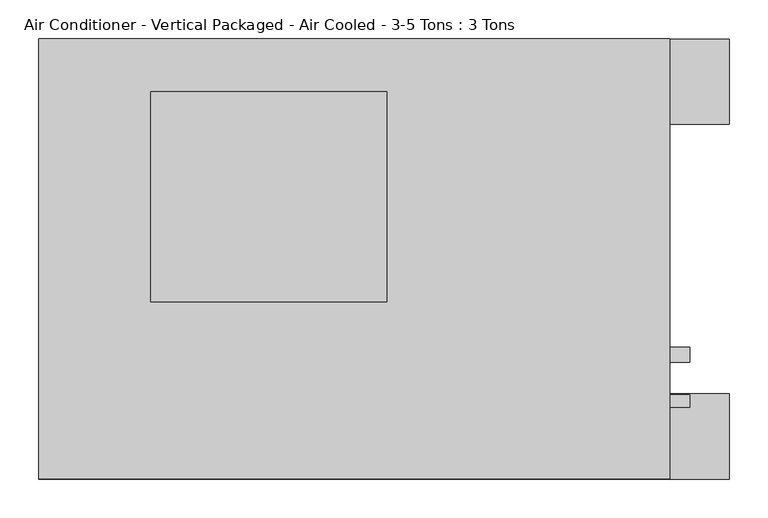
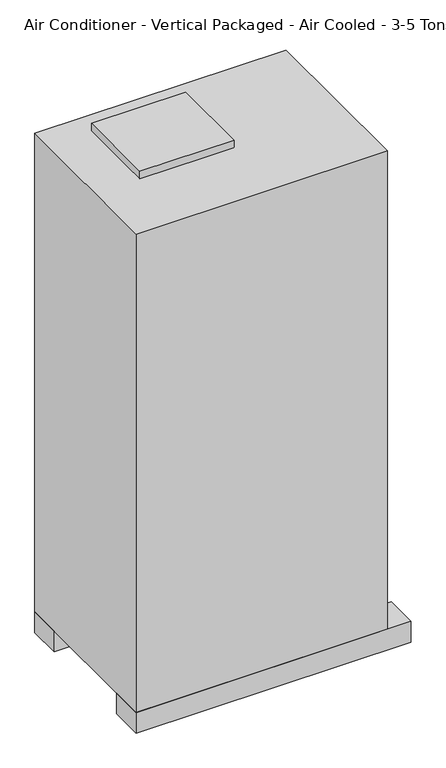
"""IFC4 building model written with IfcOpenShell, lengths in millimetres: proxy geometry, Air Conditioner - Vertical Packaged - Air Cooled - 3-5 Tons : 3 Tons."""

import ifcopenshell
import ifcopenshell.guid

model = None  # the IFC model being written
_history = None  # IfcOwnerHistory: only IFC2X3 demands one
_inside = {}  # id of a spatial element -> (the spatial element, [elements in it])
_under = {}  # id of a project, library or spatial element -> (it, [spatial elements below it])
_declared = {}  # id of a project -> (the project, [libraries it declares])
_typed = {}  # id of a type object -> (the type object, [elements of that type])
_made_of = {}  # id of a material, layer set ... -> (it, [elements and type objects made of it])


def new_model(schema):
    """Start an empty IFC model of exactly this schema.

    Asked for "IFC4X3", IfcOpenShell would pick the latest addendum, in which some entities
    have other attributes; the version numbers below select the first issue.
    IFC2X3 requires an IfcOwnerHistory on every rooted entity: one is made here for all.
    """
    global model, _history
    if schema == "IFC4X3":
        model = ifcopenshell.file(schema_version=(4, 3, 0, 0))
    else:
        model = ifcopenshell.file(schema=schema)
    _inside.clear()
    _under.clear()
    _declared.clear()
    _typed.clear()
    _made_of.clear()
    _history = None
    if model.schema == "IFC2X3":
        org = make("IfcOrganization", Name="unknown")
        user = make(
            "IfcPersonAndOrganization",
            ThePerson=make("IfcPerson", FamilyName="unknown"),
            TheOrganization=org,
        )
        app = make(
            "IfcApplication",
            ApplicationDeveloper=org,
            Version="unknown",
            ApplicationFullName="unknown",
            ApplicationIdentifier="unknown",
        )
        _history = make(
            "IfcOwnerHistory",
            OwningUser=user,
            OwningApplication=app,
            ChangeAction="ADDED",
            CreationDate=0,
        )
    return model


def make(cls, **values):
    """One entity of the class cls with the attributes given. An attribute that is None is left unset."""
    return model.create_entity(
        cls, **{name: value for name, value in values.items() if value is not None}
    )


def rooted(cls, **values):
    """An entity with a GlobalId (a new one), such as an element, a storey or a relation."""
    return make(cls, GlobalId=ifcopenshell.guid.new(), OwnerHistory=_history, **values)


def si_unit(unit_type, name, prefix=None):
    """IfcSIUnit, for example si_unit("LENGTHUNIT", "METRE", prefix="MILLI")."""
    return make("IfcSIUnit", UnitType=unit_type, Prefix=prefix, Name=name)


def assignment(units):
    """IfcUnitAssignment: the units of a project."""
    return None if units is None else make("IfcUnitAssignment", Units=units)


def point(xyz):
    """IfcCartesianPoint."""
    return None if xyz is None else make("IfcCartesianPoint", Coordinates=xyz)


def direction(xyz):
    """IfcDirection."""
    return None if xyz is None else make("IfcDirection", DirectionRatios=xyz)


def frame(location, z_axis=None, x_axis=None):
    """IfcAxis2Placement3D, a coordinate frame: its origin and axes. An axis left out is left unset."""
    return make(
        "IfcAxis2Placement3D",
        Location=point(location),
        Axis=direction(z_axis),
        RefDirection=direction(x_axis),
    )


def frame_2d(location, x_axis=None):
    """IfcAxis2Placement2D, a coordinate frame in the plane: its origin and x axis."""
    return make(
        "IfcAxis2Placement2D", Location=point(location), RefDirection=direction(x_axis)
    )


def origin():
    """The frame at (0, 0, 0) with its axes left unset."""
    return frame((0.0, 0.0, 0.0))


def origin_with_axes():
    """The frame at (0, 0, 0) with the z axis (0, 0, 1) and the x axis (1, 0, 0) written out."""
    return frame((0.0, 0.0, 0.0), z_axis=(0.0, 0.0, 1.0), x_axis=(1.0, 0.0, 0.0))


def place(relative_to, where):
    """IfcLocalPlacement: puts the frame where relative to a parent placement (None: the world)."""
    return make(
        "IfcLocalPlacement", PlacementRelTo=relative_to, RelativePlacement=where
    )


def context(
    kind, dimensions, precision=None, world=None, true_north=None, identifier=None
):
    """IfcGeometricRepresentationContext, for example the 3D "Model" context."""
    return make(
        "IfcGeometricRepresentationContext",
        ContextIdentifier=identifier,
        ContextType=kind,
        CoordinateSpaceDimension=dimensions,
        Precision=precision,
        WorldCoordinateSystem=world,
        TrueNorth=true_north,
    )


def project(units=None, contexts=None):
    """IfcProject with its units and contexts."""
    return rooted(
        "IfcProject",
        Name="project",
        RepresentationContexts=contexts,
        UnitsInContext=assignment(units),
    )


def spatial(cls, under=None, at=None, **own):
    """A site, building, storey or space (cls), placed at a placement, below another one or the project."""
    s = rooted(cls, ObjectPlacement=at, **own)
    if under is not None:
        _under.setdefault(under.id(), (under, []))[1].append(s)
    return s


def polyline(points):
    """IfcPolyline through the points."""
    return make("IfcPolyline", Points=[point(p) for p in points])


def circle_curve(where, radius):
    """IfcCircle in the frame where."""
    return make("IfcCircle", Position=where, Radius=radius)


def trimmed(basis, trim1, trim2, sense, master):
    """IfcTrimmedCurve: the piece of a basis curve between two trims."""
    return make(
        "IfcTrimmedCurve",
        BasisCurve=basis,
        Trim1=trim1,
        Trim2=trim2,
        SenseAgreement=sense,
        MasterRepresentation=master,
    )


def segment(curve, same_sense, transition):
    """IfcCompositeCurveSegment."""
    return make(
        "IfcCompositeCurveSegment",
        Transition=transition,
        SameSense=same_sense,
        ParentCurve=curve,
    )


def composite_curve(segments, self_intersect=None):
    """IfcCompositeCurve: segments joined end to end."""
    return make("IfcCompositeCurve", Segments=segments, SelfIntersect=self_intersect)


def outline(outer, holes=None, kind="AREA"):
    """IfcArbitraryClosedProfileDef: a profile drawn as a closed curve; with holes, ...WithVoids."""
    if holes is None:
        return make("IfcArbitraryClosedProfileDef", ProfileType=kind, OuterCurve=outer)
    return make(
        "IfcArbitraryProfileDefWithVoids",
        ProfileType=kind,
        OuterCurve=outer,
        InnerCurves=holes,
    )


def extrude(swept, where, along, depth):
    """IfcExtrudedAreaSolid: the profile swept, set in the frame where, extruded along a direction by depth."""
    return make(
        "IfcExtrudedAreaSolid",
        SweptArea=swept,
        Position=where,
        ExtrudedDirection=direction(along),
        Depth=depth,
    )


def shape(context_of_items, identifier, shape_type, items):
    """IfcShapeRepresentation: the items that make up one representation, for example the "Body"."""
    return make(
        "IfcShapeRepresentation",
        ContextOfItems=context_of_items,
        RepresentationIdentifier=identifier,
        RepresentationType=shape_type,
        Items=items,
    )


def source(mapping_origin, context_of_items, identifier, shape_type, items):
    """IfcRepresentationMap: a shape defined once, which mapped items show again and again."""
    return make(
        "IfcRepresentationMap",
        MappingOrigin=mapping_origin,
        MappedRepresentation=shape(context_of_items, identifier, shape_type, items),
    )


def transform(
    local_origin,
    x_axis=None,
    y_axis=None,
    z_axis=None,
    scale=None,
    scale2=None,
    scale3=None,
    uniform=True,
):
    """IfcCartesianTransformationOperator3D, or its non-uniform kind. x_axis, y_axis, z_axis: its Axis1, 2, 3."""
    if uniform:
        return make(
            "IfcCartesianTransformationOperator3D",
            Axis1=direction(x_axis),
            Axis2=direction(y_axis),
            LocalOrigin=point(local_origin),
            Scale=scale,
            Axis3=direction(z_axis),
        )
    return make(
        "IfcCartesianTransformationOperator3DnonUniform",
        Axis1=direction(x_axis),
        Axis2=direction(y_axis),
        LocalOrigin=point(local_origin),
        Scale=scale,
        Axis3=direction(z_axis),
        Scale2=scale2,
        Scale3=scale3,
    )


def mapped(mapping_source, mapping_target):
    """IfcMappedItem: shows the shape of a source again, moved by a transform."""
    return make(
        "IfcMappedItem", MappingSource=mapping_source, MappingTarget=mapping_target
    )


def made_of(thing, what):
    """Note that an element or type object is made of a material, layer set ...; save() writes the relation."""
    if what is not None:
        _made_of.setdefault(what.id(), (what, []))[1].append(thing)
    return thing


def element(
    cls,
    number,
    at=None,
    inside=None,
    cuts=None,
    type_object=None,
    material=None,
    context=None,
    identifier="Body",
    shape_type=None,
    held_by="IfcProductDefinitionShape",
    body=None,
    shapes=None,
    **own,
):
    """One element of the class cls, such as IfcWall. Its Tag is "e" and its number.

    at: its placement. inside: the storey or other place that contains it. cuts: it is an
    opening in that element (IfcRelVoidsElement). A single representation is given by context,
    identifier, shape_type and body (its items); several are given by shapes. held_by: the class
    of the entity that holds the representations. save() writes the other relations.
    """
    e = rooted(cls, Tag="e%d" % number, ObjectPlacement=at, **own)
    if body is not None:
        shapes = [shape(context, identifier, shape_type, body)]
    if shapes is not None:
        e.Representation = make(held_by, Representations=shapes)
    if inside is not None:
        _inside.setdefault(inside.id(), (inside, []))[1].append(e)
    if cuts is not None:
        rooted(
            "IfcRelVoidsElement", RelatingBuildingElement=cuts, RelatedOpeningElement=e
        )
    if type_object is not None:
        _typed.setdefault(type_object.id(), (type_object, []))[1].append(e)
    return made_of(e, material)


def aggregate(whole, parts):
    """IfcRelAggregates: a whole, such as a stair, and the parts it consists of."""
    return rooted("IfcRelAggregates", RelatingObject=whole, RelatedObjects=parts)


def save(model, path):
    """Write the relations noted so far, then the file.

    IfcRelAggregates (storeys below a building ...), IfcRelContainedInSpatialStructure (elements
    in a storey), IfcRelDefinesByType, IfcRelAssociatesMaterial and IfcRelDeclares: one each for
    every whole, place, type object, material and project.
    """
    for whole, parts in _under.values():
        aggregate(whole, parts)
    for where, things in _inside.values():
        rooted(
            "IfcRelContainedInSpatialStructure",
            RelatedElements=things,
            RelatingStructure=where,
        )
    for kind, things in _typed.values():
        rooted("IfcRelDefinesByType", RelatedObjects=things, RelatingType=kind)
    for what, things in _made_of.values():
        rooted("IfcRelAssociatesMaterial", RelatedObjects=things, RelatingMaterial=what)
    for by, libraries in _declared.values():
        rooted("IfcRelDeclares", RelatingContext=by, RelatedDefinitions=libraries)
    model.write(path)


def air_conditioner_vertical_packaged_air_cooled_3_5_tons_3_tons_b39a03d3(model_context):
    return source(origin(), model_context, "Body", "SweptSolid", [
        extrude(outline(composite_curve([segment(trimmed(circle_curve(frame_2d((159.54375, 513.0601562)), 9.525), [point((150.01875, 513.0601562))], [point((169.06875, 513.0601562))], False, "CARTESIAN"), True, "CONTINUOUS"), segment(trimmed(circle_curve(frame_2d((159.54375, 513.0601562)), 9.525), [point((169.06875, 513.0601562))], [point((150.01875, 513.0601562))], False, "CARTESIAN"), True, "CONTINUOUS")], self_intersect=False)), frame((810.021875, 0.0, 0.0), z_axis=(1.0, 0.0, 0.0), x_axis=(0.0, 1.0, 0.0)), (0.0, 0.0, 1.0), 25.4),
        extrude(outline(polyline([(446.484375, 497.0343437), (446.484375, 227.060125), (143.4703125, 227.060125), (143.4703125, 497.0343437), (446.484375, 497.0343437)])), frame((0.0, 0.0, 1700.069625), z_axis=(0.0, 0.0, 1.0), x_axis=(1.0, 0.0, 0.0)), (0.0, 0.0, 1.0), 25.4),
        extrude(outline(composite_curve([segment(trimmed(circle_curve(frame_2d((454.3226562, 330.9500937)), 12.7), [point((441.6226562, 330.9500937))], [point((467.0226562, 330.9500937))], False, "CARTESIAN"), True, "CONTINUOUS"), segment(trimmed(circle_curve(frame_2d((454.3226562, 330.9500937)), 12.7), [point((467.0226562, 330.9500937))], [point((441.6226562, 330.9500937))], False, "CARTESIAN"), True, "CONTINUOUS")], self_intersect=False)), frame((784.621875, 0.0, 0.0), z_axis=(1.0, 0.0, 0.0), x_axis=(0.0, 1.0, 0.0)), (0.0, 0.0, 1.0), 25.4),
        extrude(outline(composite_curve([segment(trimmed(circle_curve(frame_2d((100.1117188, 170.2157187)), 6.35), [point((93.7617188, 170.2157187))], [point((106.4617188, 170.2157187))], False, "CARTESIAN"), True, "CONTINUOUS"), segment(trimmed(circle_curve(frame_2d((100.1117188, 170.2157187)), 6.35), [point((106.4617188, 170.2157187))], [point((93.7617188, 170.2157187))], False, "CARTESIAN"), True, "CONTINUOUS")], self_intersect=False)), frame((810.021875, 0.0, 0.0), z_axis=(1.0, 0.0, 0.0), x_axis=(0.0, 1.0, 0.0)), (0.0, 0.0, 1.0), 25.4),
        extrude(outline(composite_curve([segment(trimmed(circle_curve(frame_2d((100.1117188, 225.0836875)), 7.9375), [point((92.1742188, 225.0836875))], [point((108.0492188, 225.0836875))], False, "CARTESIAN"), True, "CONTINUOUS"), segment(trimmed(circle_curve(frame_2d((100.1117188, 225.0836875)), 7.9375), [point((108.0492188, 225.0836875))], [point((92.1742188, 225.0836875))], False, "CARTESIAN"), True, "CONTINUOUS")], self_intersect=False)), frame((810.021875, 0.0, 0.0), z_axis=(1.0, 0.0, 0.0), x_axis=(0.0, 1.0, 0.0)), (0.0, 0.0, 1.0), 25.4),
        extrude(outline(polyline([(886.221875, 109.22), (886.221875, 0.0), (0.0, 0.0), (0.0, 109.22), (886.221875, 109.22)])), origin_with_axes(), (0.0, 0.0, 1.0), 70.104),
        extrude(outline(polyline([(886.221875, 564.8523437), (886.221875, 455.6323437), (0.0, 455.6323437), (0.0, 564.8523437), (886.221875, 564.8523437)])), origin_with_axes(), (0.0, 0.0, 1.0), 70.104),
        extrude(outline(polyline([(810.021875, 564.8523437), (810.021875, 0.0), (0.0, 0.0), (0.0, 564.8523437), (810.021875, 564.8523437)])), frame((0.0, 0.0, 70.104), z_axis=(0.0, 0.0, 1.0), x_axis=(1.0, 0.0, 0.0)), (0.0, 0.0, 1.0), 1629.965625),
    ])


if __name__ == "__main__":
    model = new_model("IFC4")
    model_context = context("Model", 3, world=origin())
    ifc_project = project(units=[si_unit("LENGTHUNIT", "METRE", prefix="MILLI")], contexts=[model_context])
    site = spatial("IfcSite", under=ifc_project)
    building = spatial("IfcBuilding", under=site)
    placement = place(None, origin())
    air_conditioner_vertical_packaged_air_cooled_3_5_tons_3_tons_shape = air_conditioner_vertical_packaged_air_cooled_3_5_tons_3_tons_b39a03d3(model_context)
    element("IfcBuildingElementProxy", 1, Name="Air Conditioner - Vertical Packaged - Air Cooled - 3-5 Tons : 3 Tons", ObjectType="Air Conditioner - Vertical Packaged - Air Cooled - 3-5 Tons : 3 Tons", at=placement, inside=building, context=model_context, shape_type="MappedRepresentation", body=[
        mapped(air_conditioner_vertical_packaged_air_cooled_3_5_tons_3_tons_shape, transform((0.0, 0.0, 0.0), x_axis=(1.0, 0.0, 0.0), y_axis=(0.0, 1.0, 0.0), z_axis=(0.0, 0.0, 1.0))),
    ])
    save(model, "model.ifc")

# Revit data of these elements
# Type "Air Conditioner - Vertical Packaged - Air Cooled - 3-5 Tons : 3 Tons"
#   Voltage = 460 V
#   Outlet Radius = 5/16"
#   Outlet Diameter = 5/8"
#   Inlet Radius = 1/4"
#   Inlet Diameter = 1/2"
#   Height 1 = 1' - 3 77/128"
#   Duct Width = 11 119/128"
#   Duct Height = 10 161/256"
#   Drain Radius = 3/8"
#   Drain Flow [instance default] = 0 GPM
#   Conditioner Width = 1' - 10 61/256"
#   Conditioner Length = 2' - 7 57/64"
#   Conditioner Height = 5' - 4 11/64"
#   C5 Offset 2 = 0' - 6 9/32"
#   C5 Offset 1 = 1' - 8 51/256"
#   C3 Offset 1 = 0' - 5 83/128"
#   C4 Offset 2 = 0' - 10 69/256"
#   C4 Offset 1 = 0' - 4 45/128"
#   C2 Offset 2 = 0' - 2 41/256"
#   C1 Offset 2 = 0' - 3 241/256"
#   C1 Offset 1 = 0' - 3 241/256"
#   Apparent Load = 6000 VA
#   Air Flow [instance default] = 1200 CFM
#   Number of Poles = 3
#   Material = none
#   Load Classification = Cooling
#   Default Elevation = 0
